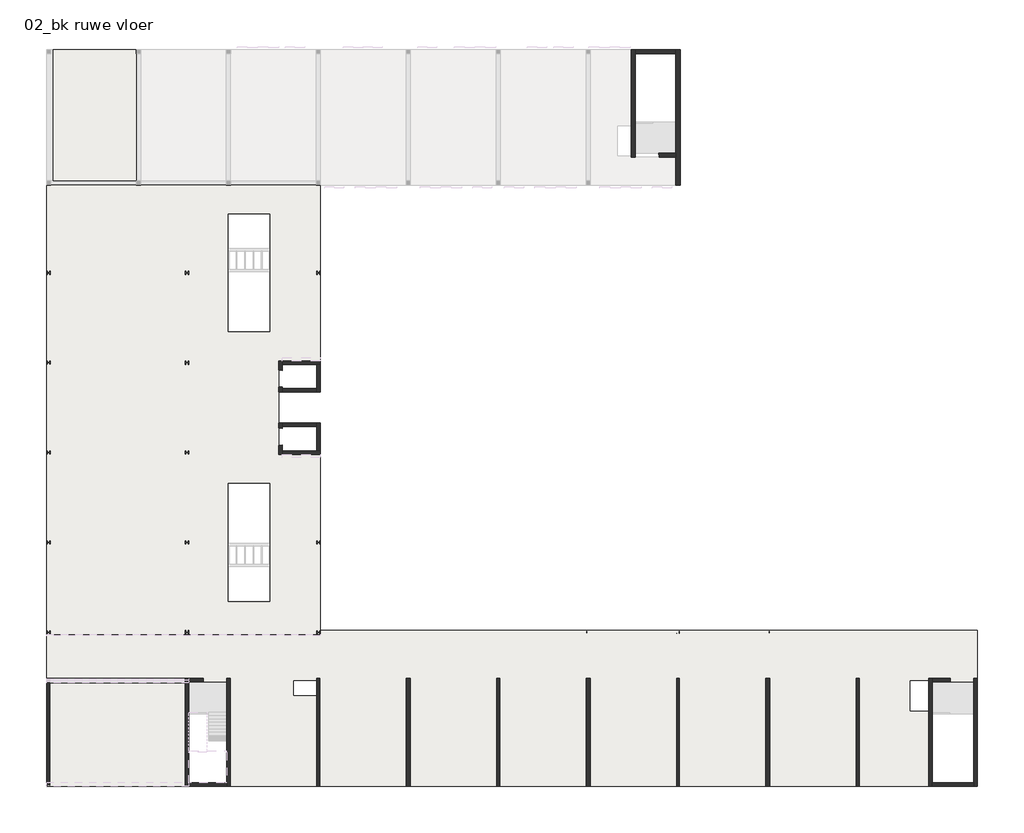
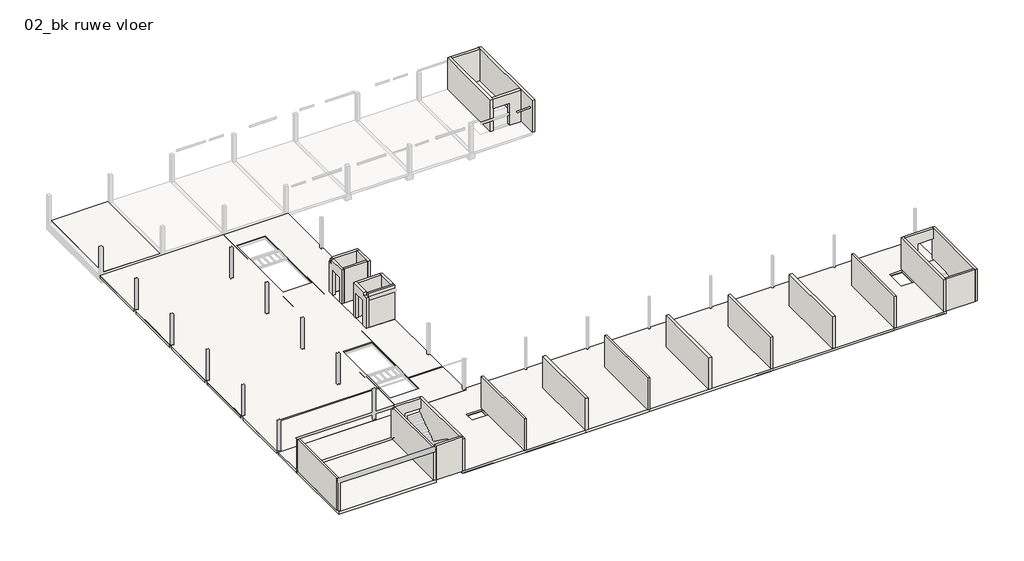
# One storey, part 1 of 3: 28 walls, 20 slabs.
"""IFC4 building model written with IfcOpenShell, lengths in millimetres."""

import ifcopenshell
import ifcopenshell.guid

model = None  # the IFC model being written
_history = None  # IfcOwnerHistory: only IFC2X3 demands one
_inside = {}  # id of a spatial element -> (the spatial element, [elements in it])
_under = {}  # id of a project, library or spatial element -> (it, [spatial elements below it])
_declared = {}  # id of a project -> (the project, [libraries it declares])
_typed = {}  # id of a type object -> (the type object, [elements of that type])
_made_of = {}  # id of a material, layer set ... -> (it, [elements and type objects made of it])


def new_model(schema):
    """Start an empty IFC model of exactly this schema.

    Asked for "IFC4X3", IfcOpenShell would pick the latest addendum, in which some entities
    have other attributes; the version numbers below select the first issue.
    IFC2X3 requires an IfcOwnerHistory on every rooted entity: one is made here for all.
    """
    global model, _history
    if schema == "IFC4X3":
        model = ifcopenshell.file(schema_version=(4, 3, 0, 0))
    else:
        model = ifcopenshell.file(schema=schema)
    _inside.clear()
    _under.clear()
    _declared.clear()
    _typed.clear()
    _made_of.clear()
    _history = None
    if model.schema == "IFC2X3":
        org = make("IfcOrganization", Name="unknown")
        user = make(
            "IfcPersonAndOrganization",
            ThePerson=make("IfcPerson", FamilyName="unknown"),
            TheOrganization=org,
        )
        app = make(
            "IfcApplication",
            ApplicationDeveloper=org,
            Version="unknown",
            ApplicationFullName="unknown",
            ApplicationIdentifier="unknown",
        )
        _history = make(
            "IfcOwnerHistory",
            OwningUser=user,
            OwningApplication=app,
            ChangeAction="ADDED",
            CreationDate=0,
        )
    return model


def make(cls, **values):
    """One entity of the class cls with the attributes given. An attribute that is None is left unset."""
    return model.create_entity(
        cls, **{name: value for name, value in values.items() if value is not None}
    )


def rooted(cls, **values):
    """An entity with a GlobalId (a new one), such as an element, a storey or a relation."""
    return make(cls, GlobalId=ifcopenshell.guid.new(), OwnerHistory=_history, **values)


def si_unit(unit_type, name, prefix=None):
    """IfcSIUnit, for example si_unit("LENGTHUNIT", "METRE", prefix="MILLI")."""
    return make("IfcSIUnit", UnitType=unit_type, Prefix=prefix, Name=name)


def assignment(units):
    """IfcUnitAssignment: the units of a project."""
    return None if units is None else make("IfcUnitAssignment", Units=units)


def point(xyz):
    """IfcCartesianPoint."""
    return None if xyz is None else make("IfcCartesianPoint", Coordinates=xyz)


def direction(xyz):
    """IfcDirection."""
    return None if xyz is None else make("IfcDirection", DirectionRatios=xyz)


def frame(location, z_axis=None, x_axis=None):
    """IfcAxis2Placement3D, a coordinate frame: its origin and axes. An axis left out is left unset."""
    return make(
        "IfcAxis2Placement3D",
        Location=point(location),
        Axis=direction(z_axis),
        RefDirection=direction(x_axis),
    )


def origin():
    """The frame at (0, 0, 0) with its axes left unset."""
    return frame((0.0, 0.0, 0.0))


def place(relative_to, where):
    """IfcLocalPlacement: puts the frame where relative to a parent placement (None: the world)."""
    return make(
        "IfcLocalPlacement", PlacementRelTo=relative_to, RelativePlacement=where
    )


def context(
    kind, dimensions, precision=None, world=None, true_north=None, identifier=None
):
    """IfcGeometricRepresentationContext, for example the 3D "Model" context."""
    return make(
        "IfcGeometricRepresentationContext",
        ContextIdentifier=identifier,
        ContextType=kind,
        CoordinateSpaceDimension=dimensions,
        Precision=precision,
        WorldCoordinateSystem=world,
        TrueNorth=true_north,
    )


def project(units=None, contexts=None):
    """IfcProject with its units and contexts."""
    return rooted(
        "IfcProject",
        Name="project",
        RepresentationContexts=contexts,
        UnitsInContext=assignment(units),
    )


def spatial(cls, under=None, at=None, **own):
    """A site, building, storey or space (cls), placed at a placement, below another one or the project."""
    s = rooted(cls, ObjectPlacement=at, **own)
    if under is not None:
        _under.setdefault(under.id(), (under, []))[1].append(s)
    return s


def polyline(points):
    """IfcPolyline through the points."""
    return make("IfcPolyline", Points=[point(p) for p in points])


def outline(outer, holes=None, kind="AREA"):
    """IfcArbitraryClosedProfileDef: a profile drawn as a closed curve; with holes, ...WithVoids."""
    if holes is None:
        return make("IfcArbitraryClosedProfileDef", ProfileType=kind, OuterCurve=outer)
    return make(
        "IfcArbitraryProfileDefWithVoids",
        ProfileType=kind,
        OuterCurve=outer,
        InnerCurves=holes,
    )


def extrude(swept, where, along, depth):
    """IfcExtrudedAreaSolid: the profile swept, set in the frame where, extruded along a direction by depth."""
    return make(
        "IfcExtrudedAreaSolid",
        SweptArea=swept,
        Position=where,
        ExtrudedDirection=direction(along),
        Depth=depth,
    )


def faces_of(points, faces, orient=None, outer=None):
    """IfcFace entities. A face is a list of loops; a loop is a list of indices into points, from 0.

    orient and outer hold one flag for each loop. By default every Orientation is true, the
    first loop of a face is its IfcFaceOuterBound and the others are IfcFaceBound.
    """
    made = []
    for i, loops in enumerate(faces):
        bounds = []
        for j, loop in enumerate(loops):
            is_outer = j == 0 if outer is None else outer[i][j]
            bounds.append(
                make(
                    "IfcFaceOuterBound" if is_outer else "IfcFaceBound",
                    Bound=make("IfcPolyLoop", Polygon=[points[k] for k in loop]),
                    Orientation=True if orient is None else orient[i][j],
                )
            )
        made.append(make("IfcFace", Bounds=bounds))
    return made


def faceted_brep(points, faces, orient=None, outer=None, voids=None):
    """IfcFacetedBrep: a solid bounded by flat faces; with voids (closed shells), ...WithVoids."""
    shared = [point(p) for p in points]
    hull = make("IfcClosedShell", CfsFaces=faces_of(shared, faces, orient, outer))
    if voids is None:
        return make("IfcFacetedBrep", Outer=hull)
    return make(
        "IfcFacetedBrepWithVoids",
        Outer=hull,
        Voids=[
            make(cls, CfsFaces=faces_of(shared, fs, o, b)) for cls, fs, o, b in voids
        ],
    )


def shape(context_of_items, identifier, shape_type, items):
    """IfcShapeRepresentation: the items that make up one representation, for example the "Body"."""
    return make(
        "IfcShapeRepresentation",
        ContextOfItems=context_of_items,
        RepresentationIdentifier=identifier,
        RepresentationType=shape_type,
        Items=items,
    )


def made_of(thing, what):
    """Note that an element or type object is made of a material, layer set ...; save() writes the relation."""
    if what is not None:
        _made_of.setdefault(what.id(), (what, []))[1].append(thing)
    return thing


def element(
    cls,
    number,
    at=None,
    inside=None,
    cuts=None,
    type_object=None,
    material=None,
    context=None,
    identifier="Body",
    shape_type=None,
    held_by="IfcProductDefinitionShape",
    body=None,
    shapes=None,
    **own,
):
    """One element of the class cls, such as IfcWall. Its Tag is "e" and its number.

    at: its placement. inside: the storey or other place that contains it. cuts: it is an
    opening in that element (IfcRelVoidsElement). A single representation is given by context,
    identifier, shape_type and body (its items); several are given by shapes. held_by: the class
    of the entity that holds the representations. save() writes the other relations.
    """
    e = rooted(cls, Tag="e%d" % number, ObjectPlacement=at, **own)
    if body is not None:
        shapes = [shape(context, identifier, shape_type, body)]
    if shapes is not None:
        e.Representation = make(held_by, Representations=shapes)
    if inside is not None:
        _inside.setdefault(inside.id(), (inside, []))[1].append(e)
    if cuts is not None:
        rooted(
            "IfcRelVoidsElement", RelatingBuildingElement=cuts, RelatedOpeningElement=e
        )
    if type_object is not None:
        _typed.setdefault(type_object.id(), (type_object, []))[1].append(e)
    return made_of(e, material)


def aggregate(whole, parts):
    """IfcRelAggregates: a whole, such as a stair, and the parts it consists of."""
    return rooted("IfcRelAggregates", RelatingObject=whole, RelatedObjects=parts)


def save(model, path):
    """Write the relations noted so far, then the file.

    IfcRelAggregates (storeys below a building ...), IfcRelContainedInSpatialStructure (elements
    in a storey), IfcRelDefinesByType, IfcRelAssociatesMaterial and IfcRelDeclares: one each for
    every whole, place, type object, material and project.
    """
    for whole, parts in _under.values():
        aggregate(whole, parts)
    for where, things in _inside.values():
        rooted(
            "IfcRelContainedInSpatialStructure",
            RelatedElements=things,
            RelatingStructure=where,
        )
    for kind, things in _typed.values():
        rooted("IfcRelDefinesByType", RelatedObjects=things, RelatingType=kind)
    for what, things in _made_of.values():
        rooted("IfcRelAssociatesMaterial", RelatedObjects=things, RelatingMaterial=what)
    for by, libraries in _declared.values():
        rooted("IfcRelDeclares", RelatingContext=by, RelatedDefinitions=libraries)
    model.write(path)


model = new_model("IFC4")

# Units and contexts
model_context = context("Model", 3, world=origin())
ifc_project = project(units=[si_unit("LENGTHUNIT", "METRE", prefix="MILLI")], contexts=[model_context])

# Site, building, storey
site = spatial("IfcSite", under=ifc_project)
building = spatial("IfcBuilding", under=site)
storey = spatial("IfcBuildingStorey", under=building, Name="02_bk ruwe vloer", Elevation=7530.0)

# Slabs
placement = place(None, origin())
element("IfcSlab", 1, ObjectType="NLRS_23_FL_breedplaat 260_gen_rsf", at=placement, inside=storey, context=model_context, shape_type="Brep", body=[
    faceted_brep([(70375.0, -150.0, 7270.0), (70125.0, -150.0, 7270.0), (65150.0, -150.0, 7270.0), (64850.0, -150.0, 7270.0), (58650.0, -150.0, 7270.0), (58350.0, -150.0, 7270.0), (52150.0, -150.0, 7270.0), (51850.0, -150.0, 7270.0), (45650.0, -150.0, 7270.0), (45350.0, -150.0, 7270.0), (39150.0, -150.0, 7270.0), (38850.0, -150.0, 7270.0), (32650.0, -150.0, 7270.0), (32350.0, -150.0, 7270.0), (19625.0, -150.0, 7270.0), (19375.0, -150.0, 7270.0), (19375.0, 7400.0, 7270.0), (16625.0, 7400.0, 7270.0), (16625.0, 7493.0, 7270.0), (16625.0, 7507.0, 7270.0), (6350.0, 7507.0, 7270.0), (6350.0, 10845.0, 7270.0), (26125.0, 10845.0, 7270.0), (26125.0, 11125.0, 7270.0), (73650.0, 11125.0, 7270.0), (73650.0, 7400.0, 7270.0), (73400.0, 7400.0, 7270.0), (70375.0, 7400.0, 7270.0), (6370.0, 7622.0, 7270.0), (19600.0, 7622.0, 7270.0), (19600.0, -130.0, 7270.0), (25875.0, -130.0, 7270.0), (25875.0, 7625.0, 7270.0), (26125.0, 7625.0, 7270.0), (26125.0, -130.0, 7270.0), (32375.0, -130.0, 7270.0), (32375.0, 125.0, 7270.0), (32625.0, 125.0, 7270.0), (32625.0, -130.0, 7270.0), (38875.0, -130.0, 7270.0), (38875.0, 7625.0, 7270.0), (39125.0, 7625.0, 7270.0), (39125.0, -130.0, 7270.0), (45375.0, -130.0, 7270.0), (45375.0, 125.0, 7270.0), (45625.0, 125.0, 7270.0), (45625.0, -130.0, 7270.0), (51875.0, -130.0, 7270.0), (51875.0, 7625.0, 7270.0), (52125.0, 7625.0, 7270.0), (52125.0, -130.0, 7270.0), (58375.0, -130.0, 7270.0), (58375.0, 125.0, 7270.0), (58625.0, 125.0, 7270.0), (58625.0, -130.0, 7270.0), (64875.0, -130.0, 7270.0), (64875.0, 7625.0, 7270.0), (65125.0, 7625.0, 7270.0), (65125.0, -130.0, 7270.0), (70150.0, -130.0, 7270.0), (70150.0, 7625.0, 7270.0), (73630.0, 7625.0, 7270.0), (73630.0, 11105.0, 7270.0), (26145.0, 11105.0, 7270.0), (26145.0, 10761.5, 7270.0), (6370.0, 10761.5, 7270.0), (32375.0, 7625.0, 7270.0), (32625.0, 7625.0, 7270.0), (32625.0, 7375.0, 7270.0), (32375.0, 7375.0, 7270.0), (45375.0, 7625.0, 7270.0), (45625.0, 7625.0, 7270.0), (45625.0, 7375.0, 7270.0), (45375.0, 7375.0, 7270.0), (58375.0, 7625.0, 7270.0), (58625.0, 7625.0, 7270.0), (58625.0, 7375.0, 7270.0), (58375.0, 7375.0, 7270.0), (19375.0, -150.0, 7530.0), (19625.0, -150.0, 7530.0), (32350.0, -150.0, 7530.0), (32650.0, -150.0, 7530.0), (45350.0, -150.0, 7530.0), (45650.0, -150.0, 7530.0), (58350.0, -150.0, 7530.0), (58650.0, -150.0, 7530.0), (70125.0, -150.0, 7530.0), (70375.0, -150.0, 7530.0), (70375.0, 7400.0, 7530.0), (71700.0, 7400.0, 7530.0), (73650.0, 7400.0, 7530.0), (73650.0, 11125.0, 7530.0), (26125.0, 11125.0, 7530.0), (26125.0, 10845.0, 7530.0), (6350.0, 10845.0, 7530.0), (6350.0, 7507.0, 7530.0), (16625.0, 7507.0, 7530.0), (16625.0, 7493.0, 7530.0), (16625.0, 7400.0, 7530.0), (19375.0, 7400.0, 7530.0), (19375.0, 100.0, 7530.0), (24227.5, 6452.0, 7530.0), (24227.5, 7500.0, 7530.0), (25850.0, 7500.0, 7530.0), (25850.0, 6452.0, 7530.0), (68805.0, 5320.0, 7530.0), (68805.0, 7500.0, 7530.0), (70125.0, 7500.0, 7530.0), (70125.0, 5320.0, 7530.0), (6350.0, 10845.0, 7480.0), (26125.0, 10845.0, 7480.0), (19600.0, 7622.0, 7330.0), (6370.0, 7622.0, 7330.0), (6370.0, 10761.5, 7330.0), (26145.0, 10761.5, 7330.0), (26145.0, 11105.0, 7330.0), (73630.0, 11105.0, 7330.0), (73630.0, 7625.0, 7330.0), (70150.0, 7625.0, 7330.0), (70150.0, -130.0, 7330.0), (65125.0, -130.0, 7330.0), (65125.0, 7625.0, 7330.0), (64875.0, 7625.0, 7330.0), (64875.0, -130.0, 7330.0), (58625.0, -130.0, 7330.0), (58625.0, 125.0, 7330.0), (58375.0, 125.0, 7330.0), (58375.0, -130.0, 7330.0), (52125.0, -130.0, 7330.0), (52125.0, 7625.0, 7330.0), (51875.0, 7625.0, 7330.0), (51875.0, -130.0, 7330.0), (45625.0, -130.0, 7330.0), (45625.0, 125.0, 7330.0), (45375.0, 125.0, 7330.0), (45375.0, -130.0, 7330.0), (39125.0, -130.0, 7330.0), (39125.0, 7625.0, 7330.0), (38875.0, 7625.0, 7330.0), (38875.0, -130.0, 7330.0), (32625.0, -130.0, 7330.0), (32625.0, 125.0, 7330.0), (32375.0, 125.0, 7330.0), (32375.0, -130.0, 7330.0), (26125.0, -130.0, 7330.0), (26125.0, 7625.0, 7330.0), (25875.0, 7625.0, 7330.0), (25875.0, -130.0, 7330.0), (19600.0, -130.0, 7330.0), (32625.0, 7625.0, 7330.0), (32375.0, 7625.0, 7330.0), (32375.0, 7375.0, 7330.0), (32625.0, 7375.0, 7330.0), (45625.0, 7625.0, 7330.0), (45375.0, 7625.0, 7330.0), (45375.0, 7375.0, 7330.0), (45625.0, 7375.0, 7330.0), (58625.0, 7625.0, 7330.0), (58375.0, 7625.0, 7330.0), (58375.0, 7375.0, 7330.0), (58625.0, 7375.0, 7330.0), (24227.5, 7500.0, 7330.0), (24227.5, 6452.0, 7330.0), (25850.0, 6452.0, 7330.0), (25850.0, 7500.0, 7330.0), (68805.0, 7500.0, 7330.0), (68805.0, 5320.0, 7330.0), (70125.0, 5320.0, 7330.0), (70125.0, 7500.0, 7330.0)], [[[0, 1, 2, 3, 4, 5, 6, 7, 8, 9, 10, 11, 12, 13, 14, 15, 16, 17, 18, 19, 20, 21, 22, 23, 24, 25, 26, 27], [28, 29, 30, 31, 32, 33, 34, 35, 36, 37, 38, 39, 40, 41, 42, 43, 44, 45, 46, 47, 48, 49, 50, 51, 52, 53, 54, 55, 56, 57, 58, 59, 60, 61, 62, 63, 64, 65]], [[66, 67, 68, 69]], [[70, 71, 72, 73]], [[74, 75, 76, 77]], [[78, 79, 80, 81, 82, 83, 84, 85, 86, 87, 88, 89, 90, 91, 92, 93, 94, 95, 96, 97, 98, 99, 100], [101, 102, 103, 104], [105, 106, 107, 108]], [[15, 14, 13, 12, 11, 10, 9, 8, 7, 6, 5, 4, 3, 2, 1, 0, 87, 86, 85, 84, 83, 82, 81, 80, 79, 78]], [[16, 15, 78, 100, 99]], [[17, 16, 99, 98]], [[17, 98, 97, 96, 19, 18]], [[21, 20, 95, 94, 109]], [[22, 21, 109, 94, 93, 110]], [[23, 22, 110, 93, 92]], [[24, 23, 92, 91]], [[25, 24, 91, 90]], [[27, 26, 25, 90, 89, 88]], [[0, 27, 88, 87]], [[20, 19, 96, 95]], [[111, 112, 113, 114, 115, 116, 117, 118, 119, 120, 121, 122, 123, 124, 125, 126, 127, 128, 129, 130, 131, 132, 133, 134, 135, 136, 137, 138, 139, 140, 141, 142, 143, 144, 145, 146, 147, 148], [149, 150, 151, 152], [153, 154, 155, 156], [157, 158, 159, 160], [161, 162, 163, 164], [165, 166, 167, 168]], [[112, 111, 29, 28]], [[113, 112, 28, 65]], [[114, 113, 65, 64]], [[115, 114, 64, 63]], [[116, 115, 63, 62]], [[117, 116, 62, 61]], [[118, 117, 61, 60]], [[119, 118, 60, 59]], [[120, 119, 59, 58]], [[121, 120, 58, 57]], [[122, 121, 57, 56]], [[123, 122, 56, 55]], [[124, 123, 55, 54]], [[125, 124, 54, 53]], [[126, 125, 53, 52]], [[127, 126, 52, 51]], [[128, 127, 51, 50]], [[129, 128, 50, 49]], [[130, 129, 49, 48]], [[131, 130, 48, 47]], [[132, 131, 47, 46]], [[133, 132, 46, 45]], [[134, 133, 45, 44]], [[135, 134, 44, 43]], [[136, 135, 43, 42]], [[137, 136, 42, 41]], [[138, 137, 41, 40]], [[139, 138, 40, 39]], [[140, 139, 39, 38]], [[141, 140, 38, 37]], [[142, 141, 37, 36]], [[143, 142, 36, 35]], [[144, 143, 35, 34]], [[145, 144, 34, 33]], [[146, 145, 33, 32]], [[147, 146, 32, 31]], [[148, 147, 31, 30]], [[111, 148, 30, 29]], [[150, 149, 67, 66]], [[151, 150, 66, 69]], [[152, 151, 69, 68]], [[149, 152, 68, 67]], [[154, 153, 71, 70]], [[155, 154, 70, 73]], [[156, 155, 73, 72]], [[153, 156, 72, 71]], [[158, 157, 75, 74]], [[159, 158, 74, 77]], [[160, 159, 77, 76]], [[157, 160, 76, 75]], [[102, 101, 162, 161]], [[101, 104, 163, 162]], [[104, 103, 164, 163]], [[103, 102, 161, 164]], [[106, 105, 166, 165]], [[105, 108, 167, 166]], [[108, 107, 168, 167]], [[107, 106, 165, 168]]]),
])
element("IfcSlab", 2, ObjectType="NLRS_23_FL_breedplaat 260_gen_rsf", at=placement, inside=storey, context=model_context, shape_type="Brep", body=[
    faceted_brep([(6830.0, 43680.0, 7270.0), (6830.0, 43800.0, 7270.0), (6830.0, 53150.0, 7270.0), (6950.0, 53150.0, 7270.0), (12700.0, 53150.0, 7270.0), (12820.0, 53150.0, 7270.0), (12820.0, 43800.0, 7270.0), (12820.0, 43680.0, 7270.0), (12725.0, 43775.0, 7270.0), (12725.0, 53140.0, 7270.0), (6925.0, 53140.0, 7270.0), (6925.0, 43775.0, 7270.0), (6830.0, 53150.0, 7530.0), (6830.0, 43680.0, 7530.0), (12820.0, 43680.0, 7530.0), (12820.0, 53150.0, 7530.0), (6925.0, 53140.0, 7330.0), (12725.0, 53140.0, 7330.0), (12725.0, 43775.0, 7330.0), (6925.0, 43775.0, 7330.0)], [[[0, 1, 2, 3, 4, 5, 6, 7], [8, 9, 10, 11]], [[12, 13, 14, 15]], [[2, 1, 0, 13, 12]], [[5, 4, 3, 2, 12, 15]], [[7, 6, 5, 15, 14]], [[0, 7, 14, 13]], [[16, 17, 18, 19]], [[18, 17, 9, 8]], [[19, 18, 8, 11]], [[16, 19, 11, 10]], [[17, 16, 10, 9]]]),
])
element("IfcSlab", 3, ObjectType="NLRS_23_FL_druklaag 70_gen_rsf", at=placement, inside=storey, context=model_context, shape_type="Brep", body=[
    faceted_brep([(6350.0, 43350.0, 7460.0), (26125.0, 43350.0, 7460.0), (26125.0, 43330.0, 7460.0), (26125.0, 37175.0, 7460.0), (26125.0, 37155.0, 7460.0), (22760.0, 37155.0, 7460.0), (22760.0, 36845.0, 7460.0), (26125.0, 36845.0, 7460.0), (26125.0, 36825.0, 7460.0), (26125.0, 30705.0, 7460.0), (26125.0, 30625.0, 7460.0), (23362.3, 30625.0, 7460.0), (23362.3, 30632.0, 7460.0), (6350.0, 30632.0, 7460.0), (6350.0, 30652.0, 7460.0), (6350.0, 36825.0, 7460.0), (6350.0, 36845.0, 7460.0), (19240.0, 36845.0, 7460.0), (19240.0, 37155.0, 7460.0), (6350.0, 37155.0, 7460.0), (6350.0, 37175.0, 7460.0), (6350.0, 43330.0, 7460.0), (22500.0, 32750.0, 7460.0), (22500.0, 41250.0, 7460.0), (19500.0, 41250.0, 7460.0), (19500.0, 32750.0, 7460.0), (23362.3, 23875.0, 7460.0), (26125.0, 23875.0, 7460.0), (26125.0, 23795.0, 7460.0), (26125.0, 17675.0, 7460.0), (26125.0, 17655.0, 7460.0), (26125.0, 17345.0, 7460.0), (26125.0, 17325.0, 7460.0), (26125.0, 11175.0, 7460.0), (26125.0, 11155.0, 7460.0), (6350.0, 11155.0, 7460.0), (6350.0, 11175.0, 7460.0), (6350.0, 17325.0, 7460.0), (6350.0, 17345.0, 7460.0), (19240.0, 17345.0, 7460.0), (19240.0, 17655.0, 7460.0), (6350.0, 17655.0, 7460.0), (6350.0, 17675.0, 7460.0), (6350.0, 23825.0, 7460.0), (6350.0, 23845.0, 7460.0), (19240.0, 23845.0, 7460.0), (19500.0, 23845.0, 7460.0), (22500.0, 23845.0, 7460.0), (22760.0, 23845.0, 7460.0), (23362.3, 23845.0, 7460.0), (22500.0, 21750.0, 7460.0), (19500.0, 21750.0, 7460.0), (19500.0, 13250.0, 7460.0), (22500.0, 13250.0, 7460.0), (19500.0000006, 13240.0, 7460.0), (19500.0000006, 12938.0, 7460.0), (22499.9999994, 12938.0, 7460.0), (22499.9999994, 13240.0, 7460.0), (19500.0000006, 22062.0, 7460.0), (19500.0000006, 21760.0, 7460.0), (22499.9999994, 21760.0, 7460.0), (22499.9999994, 22062.0, 7460.0), (6350.0, 30322.0, 7460.0), (23125.0, 30322.0, 7460.0), (23125.0, 30302.0, 7460.0), (23125.0, 24175.0, 7460.0), (23125.0, 24155.0, 7460.0), (6350.0, 24155.0, 7460.0), (6350.0, 24175.0, 7460.0), (6350.0, 30302.0, 7460.0), (26125.0, 30625.0, 7530.0), (26125.0, 43350.0, 7530.0), (6350.0, 43350.0, 7530.0), (6350.0, 10845.0, 7530.0), (26125.0, 10845.0, 7530.0), (26125.0, 11125.0, 7530.0), (26125.0, 23875.0, 7530.0), (23125.0, 23875.0, 7530.0), (23125.0, 30625.0, 7530.0), (22500.0, 41250.0, 7530.0), (22500.0, 32750.0, 7530.0), (19500.0, 32750.0, 7530.0), (19500.0, 41250.0, 7530.0), (19500.0, 21750.0, 7530.0), (22500.0, 21750.0, 7530.0), (22500.0, 13250.0, 7530.0), (19500.0, 13250.0, 7530.0), (26125.0, 36845.0, 7480.0), (26125.0, 37155.0, 7480.0), (6350.0, 10845.0, 7480.0), (26125.0, 10845.0, 7480.0), (6350.0, 37155.0, 7480.0), (6350.0, 36845.0, 7480.0), (6350.0, 30632.0, 7480.0), (6350.0, 30322.0, 7480.0), (6350.0, 24155.0, 7480.0), (6350.0, 23845.0, 7480.0), (6350.0, 17655.0, 7480.0), (6350.0, 17345.0, 7480.0), (6350.0, 11155.0, 7480.0), (23125.0, 30625.0, 7480.0), (23362.3, 30625.0, 7480.0), (23125.0, 23875.0, 7480.0), (23125.0, 24155.0, 7480.0), (23125.0, 30322.0, 7480.0), (23362.3, 23875.0, 7480.0), (26125.0, 11125.0, 7480.0), (26125.0, 11155.0, 7480.0), (19240.0, 36845.0, 7480.0), (19240.0, 37155.0, 7480.0), (23362.3, 30632.0, 7480.0), (23362.3, 23845.0, 7480.0), (19240.0, 17345.0, 7480.0), (19240.0, 17655.0, 7480.0), (22760.0, 37155.0, 7480.0), (22760.0, 36845.0, 7480.0), (19500.0000006, 13240.0, 7480.0), (19500.0000006, 12938.0, 7480.0), (22499.9999994, 12938.0, 7480.0), (22499.9999994, 13240.0, 7480.0), (19500.0000006, 22062.0, 7480.0), (19500.0000006, 21760.0, 7480.0), (22499.9999994, 21760.0, 7480.0), (22499.9999994, 22062.0, 7480.0)], [[[0, 1, 2, 3, 4, 5, 6, 7, 8, 9, 10, 11, 12, 13, 14, 15, 16, 17, 18, 19, 20, 21], [22, 23, 24, 25]], [[26, 27, 28, 29, 30, 31, 32, 33, 34, 35, 36, 37, 38, 39, 40, 41, 42, 43, 44, 45, 46, 47, 48, 49], [50, 51, 52, 53], [54, 55, 56, 57], [58, 59, 60, 61]], [[62, 63, 64, 65, 66, 67, 68, 69]], [[70, 71, 72, 73, 74, 75, 76, 77, 78], [79, 80, 81, 82], [83, 84, 85, 86]], [[71, 70, 10, 9, 8, 7, 87, 88, 4, 3, 2, 1]], [[74, 73, 89, 90]], [[73, 72, 0, 21, 20, 19, 91, 92, 16, 15, 14, 13, 93, 94, 62, 69, 68, 67, 95, 96, 44, 43, 42, 41, 97, 98, 38, 37, 36, 35, 99, 89]], [[1, 0, 72, 71]], [[70, 78, 100, 101, 11, 10]], [[78, 77, 102, 103, 66, 65, 64, 63, 104, 100]], [[77, 76, 27, 26, 105, 102]], [[27, 76, 75, 74, 90, 106, 107, 34, 33, 32, 31, 30, 29, 28]], [[23, 22, 80, 79]], [[24, 23, 79, 82]], [[25, 24, 82, 81]], [[22, 25, 81, 80]], [[51, 50, 84, 83]], [[52, 51, 83, 86]], [[53, 52, 86, 85]], [[50, 53, 85, 84]], [[108, 109, 18, 17]], [[109, 108, 92, 91]], [[109, 91, 19, 18]], [[92, 108, 17, 16]], [[101, 110, 12, 11]], [[93, 110, 101, 100, 104, 94]], [[110, 93, 13, 12]], [[94, 104, 63, 62]], [[111, 105, 26, 49]], [[111, 96, 95, 103, 102, 105]], [[103, 95, 67, 66]], [[96, 111, 49, 48, 47, 46, 45, 44]], [[112, 113, 40, 39]], [[113, 112, 98, 97]], [[113, 97, 41, 40]], [[98, 112, 39, 38]], [[99, 107, 106, 90, 89]], [[107, 99, 35, 34]], [[114, 115, 6, 5]], [[115, 114, 88, 87]], [[88, 114, 5, 4]], [[115, 87, 7, 6]], [[116, 117, 55, 54]], [[118, 119, 57, 56]], [[117, 116, 119, 118]], [[119, 116, 54, 57]], [[117, 118, 56, 55]], [[120, 121, 59, 58]], [[122, 123, 61, 60]], [[121, 120, 123, 122]], [[121, 122, 60, 59]], [[123, 120, 58, 61]]]),
])
element("IfcSlab", 4, ObjectType="NLRS_23_FL_kanaalplaat 260_gen_rsf", at=placement, inside=storey, context=model_context, shape_type="SweptSolid", body=[
    extrude(outline(polyline([(19240.0, 11175.0), (6350.0, 11175.0), (6350.0, 17325.0), (19240.0, 17325.0), (19240.0, 11175.0)])), frame((0.0, 0.0, 7200.0), z_axis=(0.0, 0.0, 1.0), x_axis=(1.0, 0.0, 0.0)), (0.0, 0.0, 1.0), 260.0),
])
element("IfcSlab", 5, ObjectType="NLRS_23_FL_kanaalplaat 260_gen_rsf", at=placement, inside=storey, context=model_context, shape_type="SweptSolid", body=[
    extrude(outline(polyline([(6350.0, 17675.0), (6350.0, 23825.0), (19240.0, 23825.0), (19240.0, 17675.0), (6350.0, 17675.0)])), frame((0.0, 0.0, 7200.0), z_axis=(0.0, 0.0, 1.0), x_axis=(1.0, 0.0, 0.0)), (0.0, 0.0, 1.0), 260.0),
])
element("IfcSlab", 6, ObjectType="NLRS_23_FL_kanaalplaat 260_gen_rsf", at=placement, inside=storey, context=model_context, shape_type="SweptSolid", body=[
    extrude(outline(polyline([(23125.0, 30302.0), (23125.0, 24175.0), (6350.0, 24175.0), (6350.0, 30302.0), (23125.0, 30302.0)])), frame((0.0, 0.0, 7200.0), z_axis=(0.0, 0.0, 1.0), x_axis=(1.0, 0.0, 0.0)), (0.0, 0.0, 1.0), 260.0),
])
element("IfcSlab", 7, ObjectType="NLRS_23_FL_kanaalplaat 260_gen_rsf", at=placement, inside=storey, context=model_context, shape_type="SweptSolid", body=[
    extrude(outline(polyline([(22500.0, 23825.0), (22500.0, 22082.0), (19500.0, 22082.0), (19500.0, 23825.0), (22500.0, 23825.0)])), frame((0.0, 0.0, 7200.0), z_axis=(0.0, 0.0, 1.0), x_axis=(1.0, 0.0, 0.0)), (0.0, 0.0, 1.0), 260.0),
])
element("IfcSlab", 8, ObjectType="NLRS_23_FL_kanaalplaat 260_gen_rsf", at=placement, inside=storey, context=model_context, shape_type="SweptSolid", body=[
    extrude(outline(polyline([(22500.0, 11182.5), (19500.0, 11182.5), (19500.0, 12918.0), (22500.0, 12918.0), (22500.0, 11182.5)])), frame((0.0, 0.0, 7200.0), z_axis=(0.0, 0.0, 1.0), x_axis=(1.0, 0.0, 0.0)), (0.0, 0.0, 1.0), 260.0),
])
element("IfcSlab", 9, ObjectType="NLRS_23_FL_kanaalplaat 260_gen_rsf", at=placement, inside=storey, context=model_context, shape_type="Brep", body=[
    faceted_brep([(26125.0, 23795.0, 7200.0), (26125.0, 23625.0, 7200.0), (26125.0, 17675.0, 7200.0), (22760.0, 17675.0, 7200.0), (22760.0, 23825.0, 7200.0), (23395.0, 23825.0, 7200.0), (23395.0, 23795.0, 7200.0), (26125.0, 23795.0, 7460.0), (23395.0, 23795.0, 7460.0), (23395.0, 23825.0, 7460.0), (22760.0, 23825.0, 7460.0), (22760.0, 17675.0, 7460.0), (26125.0, 17675.0, 7460.0)], [[[0, 1, 2, 3, 4, 5, 6]], [[7, 8, 9, 10, 11, 12]], [[2, 1, 0, 7, 12]], [[3, 2, 12, 11]], [[4, 3, 11, 10]], [[5, 4, 10, 9]], [[6, 5, 9, 8]], [[0, 6, 8, 7]]]),
])
element("IfcSlab", 10, ObjectType="NLRS_23_FL_kanaalplaat 260_gen_rsf", at=placement, inside=storey, context=model_context, shape_type="SweptSolid", body=[
    extrude(outline(polyline([(22760.0, 11175.0), (22760.0, 17325.0), (26125.0, 17325.0), (26125.0, 11175.0), (22760.0, 11175.0)])), frame((0.0, 0.0, 7200.0), z_axis=(0.0, 0.0, 1.0), x_axis=(1.0, 0.0, 0.0)), (0.0, 0.0, 1.0), 260.0),
])
element("IfcSlab", 11, ObjectType="NLRS_23_FL_kanaalplaat 260_gen_rsf", at=placement, inside=storey, context=model_context, shape_type="Brep", body=[
    faceted_brep([(19240.0, 43330.0, 7200.0), (19240.0, 37175.0, 7200.0), (6350.0, 37175.0, 7200.0), (6350.0, 43200.0, 7200.0), (6350.0, 43330.0, 7200.0), (19240.0, 43330.0, 7460.0), (6350.0, 43330.0, 7460.0), (6350.0, 37175.0, 7460.0), (19240.0, 37175.0, 7460.0)], [[[0, 1, 2, 3, 4]], [[5, 6, 7, 8]], [[0, 4, 6, 5]], [[4, 3, 2, 7, 6]], [[2, 1, 8, 7]], [[1, 0, 5, 8]]]),
])
element("IfcSlab", 12, ObjectType="NLRS_23_FL_kanaalplaat 260_gen_rsf", at=placement, inside=storey, context=model_context, shape_type="SweptSolid", body=[
    extrude(outline(polyline([(6350.0, 36825.0), (19240.0, 36825.0), (19240.0, 30652.0), (6350.0, 30652.0), (6350.0, 36825.0)])), frame((0.0, 0.0, 7200.0), z_axis=(0.0, 0.0, 1.0), x_axis=(1.0, 0.0, 0.0)), (0.0, 0.0, 1.0), 260.0),
])
element("IfcSlab", 13, ObjectType="NLRS_23_FL_kanaalplaat 260_gen_rsf", at=placement, inside=storey, context=model_context, shape_type="SweptSolid", body=[
    extrude(outline(polyline([(22500.0, 30652.0), (19500.0, 30652.0), (19500.0, 32418.0), (22500.0, 32418.0), (22500.0, 30652.0)])), frame((0.0, 0.0, 7200.0), z_axis=(0.0, 0.0, 1.0), x_axis=(1.0, 0.0, 0.0)), (0.0, 0.0, 1.0), 260.0),
])
element("IfcSlab", 14, ObjectType="NLRS_23_FL_kanaalplaat 260_gen_rsf", at=placement, inside=storey, context=model_context, shape_type="SweptSolid", body=[
    extrude(outline(polyline([(22500.0, 43330.0), (22500.0, 41605.0), (19500.0, 41605.0), (19500.0, 43330.0), (22500.0, 43330.0)])), frame((0.0, 0.0, 7200.0), z_axis=(0.0, 0.0, 1.0), x_axis=(1.0, 0.0, 0.0)), (0.0, 0.0, 1.0), 260.0),
])
element("IfcSlab", 15, ObjectType="NLRS_23_FL_kanaalplaat 260_gen_rsf", at=placement, inside=storey, context=model_context, shape_type="Brep", body=[
    faceted_brep([(26125.0, 30705.0, 7200.0), (23395.0, 30705.0, 7200.0), (23395.0, 30652.0, 7200.0), (22760.0, 30652.0, 7200.0), (22760.0, 36825.0, 7200.0), (26125.0, 36825.0, 7200.0), (26125.0, 30875.0, 7200.0), (26125.0, 30705.0, 7460.0), (26125.0, 36825.0, 7460.0), (22760.0, 36825.0, 7460.0), (22760.0, 30652.0, 7460.0), (23395.0, 30652.0, 7460.0), (23395.0, 30705.0, 7460.0)], [[[0, 1, 2, 3, 4, 5, 6]], [[7, 8, 9, 10, 11, 12]], [[0, 6, 5, 8, 7]], [[5, 4, 9, 8]], [[4, 3, 10, 9]], [[3, 2, 11, 10]], [[2, 1, 12, 11]], [[1, 0, 7, 12]]]),
])
element("IfcSlab", 16, ObjectType="NLRS_23_FL_kanaalplaat 260_gen_rsf", at=placement, inside=storey, context=model_context, shape_type="Brep", body=[
    faceted_brep([(22760.0, 43330.0, 7200.0), (26125.0, 43330.0, 7200.0), (26125.0, 43200.0, 7200.0), (26125.0, 37175.0, 7200.0), (22760.0, 37175.0, 7200.0), (22760.0, 43330.0, 7460.0), (22760.0, 37175.0, 7460.0), (26125.0, 37175.0, 7460.0), (26125.0, 43330.0, 7460.0)], [[[0, 1, 2, 3, 4]], [[5, 6, 7, 8]], [[0, 4, 6, 5]], [[4, 3, 7, 6]], [[3, 2, 1, 8, 7]], [[1, 0, 5, 8]]]),
])
element("IfcSlab", 17, ObjectType="NLRS_23_FL_breedplaat 260_gen_rsf", at=placement, inside=storey, context=model_context, shape_type="Brep", body=[
    faceted_brep([(6350.0, -150.0, 7270.0), (6350.0, 7493.0, 7270.0), (16625.0, 7493.0, 7270.0), (16625.0, 7330.0, 7270.0), (16625.0, 170.0, 7270.0), (16625.0, -150.0, 7270.0), (16400.0, 125.0, 7270.0), (16400.0, 7378.0, 7270.0), (6539.0, 7378.0, 7270.0), (6539.0, 125.0, 7270.0), (6350.0, 7493.0, 7530.0), (6350.0, -150.0, 7530.0), (16375.0, -150.0, 7530.0), (16625.0, -150.0, 7530.0), (16625.0, 100.0, 7530.0), (16625.0, 7493.0, 7530.0), (6539.0, 7378.0, 7330.0), (16400.0, 7378.0, 7330.0), (16400.0, 125.0, 7330.0), (6539.0, 125.0, 7330.0)], [[[0, 1, 2, 3, 4, 5], [6, 7, 8, 9]], [[10, 11, 12, 13, 14, 15]], [[1, 0, 11, 10]], [[2, 1, 10, 15]], [[5, 4, 3, 2, 15, 14, 13]], [[0, 5, 13, 12, 11]], [[16, 17, 18, 19]], [[18, 17, 7, 6]], [[19, 18, 6, 9]], [[16, 19, 9, 8]], [[17, 16, 8, 7]]]),
])
element("IfcSlab", 18, ObjectType="NLRS_23_FL_breedplaat schil 60_gen_rsf", at=placement, inside=storey, context=model_context, shape_type="SweptSolid", body=[
    extrude(outline(polyline([(19600.0, 7622.0), (6370.0, 7622.0), (6370.0, 10761.5), (26145.0, 10761.5), (26145.0, 11105.0), (73630.0, 11105.0), (73630.0, 7625.0), (70150.0, 7625.0), (70150.0, -130.0), (65125.0, -130.0), (65125.0, 7625.0), (64875.0, 7625.0), (64875.0, -130.0), (58625.0, -130.0), (58625.0, 125.0), (58375.0, 125.0), (58375.0, -130.0), (52125.0, -130.0), (52125.0, 7625.0), (51875.0, 7625.0), (51875.0, -130.0), (45625.0, -130.0), (45625.0, 125.0), (45375.0, 125.0), (45375.0, -130.0), (39125.0, -130.0), (39125.0, 7625.0), (38875.0, 7625.0), (38875.0, -130.0), (32625.0, -130.0), (32625.0, 125.0), (32375.0, 125.0), (32375.0, -130.0), (26125.0, -130.0), (26125.0, 7625.0), (25875.0, 7625.0), (25875.0, -130.0), (19600.0, -130.0), (19600.0, 7622.0)]), holes=[polyline([(32625.0, 7625.0), (32375.0, 7625.0), (32375.0, 7375.0), (32625.0, 7375.0), (32625.0, 7625.0)]), polyline([(45625.0, 7625.0), (45375.0, 7625.0), (45375.0, 7375.0), (45625.0, 7375.0), (45625.0, 7625.0)]), polyline([(58625.0, 7625.0), (58375.0, 7625.0), (58375.0, 7375.0), (58625.0, 7375.0), (58625.0, 7625.0)]), polyline([(24227.5, 7500.0), (24227.5, 6452.0), (25850.0, 6452.0), (25850.0, 7500.0), (24227.5, 7500.0)]), polyline([(68805.0, 7500.0), (68805.0, 5320.0), (70125.0, 5320.0), (70125.0, 7500.0), (68805.0, 7500.0)])]), frame((0.0, 0.0, 7270.0), z_axis=(0.0, 0.0, 1.0), x_axis=(1.0, 0.0, 0.0)), (0.0, 0.0, 1.0), 60.0),
])
element("IfcSlab", 19, ObjectType="NLRS_23_FL_breedplaat schil 60_gen_rsf", at=placement, inside=storey, context=model_context, shape_type="SweptSolid", body=[
    extrude(outline(polyline([(16400.0, 7378.0), (16400.0, 125.0), (6539.0, 125.0), (6539.0, 7378.0), (16400.0, 7378.0)])), frame((0.0, 0.0, 7270.0), z_axis=(0.0, 0.0, 1.0), x_axis=(1.0, 0.0, 0.0)), (0.0, 0.0, 1.0), 60.0),
])
element("IfcSlab", 20, ObjectType="NLRS_23_FL_breedplaat schil 60_gen_rsf", at=placement, inside=storey, context=model_context, shape_type="SweptSolid", body=[
    extrude(outline(polyline([(12725.0, 53140.0), (12725.0, 43775.0), (6925.0, 43775.0), (6925.0, 53140.0), (12725.0, 53140.0)])), frame((0.0, 0.0, 7270.0), z_axis=(0.0, 0.0, 1.0), x_axis=(1.0, 0.0, 0.0)), (0.0, 0.0, 1.0), 60.0),
])

# Walls
element("IfcWall", 21, ObjectType="NLRS_22_WA_beton ihw 250_gen_rsf", at=placement, inside=storey, context=model_context, shape_type="Brep", body=[
    faceted_brep([(19625.0, -150.0, 7530.0), (19625.0, 7650.0, 7530.0), (19625.0, 7650.0, 11070.0), (19625.0, -150.0, 11070.0), (19375.0, -150.0, 7530.0), (19375.0, -150.0, 11070.0), (19375.0, 7400.0, 11070.0), (19375.0, 7650.0, 11070.0), (19375.0, 7650.0, 9970.0), (19375.0, 7650.0, 7530.0), (19375.0, 7400.0, 7530.0), (19375.0, 100.0, 7530.0)], [[[0, 1, 2, 3]], [[4, 5, 6, 7, 8, 9, 10, 11]], [[1, 0, 4, 11, 10, 9]], [[2, 1, 9, 8, 7]], [[3, 2, 7, 6, 5]], [[0, 3, 5, 4]]]),
])
element("IfcWall", 22, ObjectType="NLRS_22_WA_beton ihw 250_gen_rsf", at=placement, inside=storey, context=model_context, shape_type="Brep", body=[
    faceted_brep([(16625.0, -150.0, 7530.0), (16625.0, 100.0, 7530.0), (16625.0, 7400.0, 7530.0), (16625.0, 7493.0, 7530.0), (16625.0, 7650.0, 7530.0), (16625.0, 7650.0, 10940.0), (16625.0, 7330.0, 10940.0), (16625.0, 7330.0, 11070.0), (16625.0, 170.0, 11070.0), (16625.0, 170.0, 10680.0), (16625.0, -150.0, 10680.0), (16375.0, -150.0, 7530.0), (16375.0, -150.0, 10680.0), (16375.0, 170.0, 10680.0), (16375.0, 170.0, 11070.0), (16375.0, 7330.0, 11070.0), (16375.0, 7330.0, 10940.0), (16375.0, 7650.0, 10940.0), (16375.0, 7650.0, 7530.0)], [[[0, 1, 2, 3, 4, 5, 6, 7, 8, 9, 10]], [[11, 12, 13, 14, 15, 16, 17, 18]], [[4, 3, 2, 1, 0, 11, 18]], [[5, 4, 18, 17]], [[8, 7, 15, 14]], [[0, 10, 12, 11]], [[9, 8, 14, 13]], [[10, 9, 13, 12]], [[6, 5, 17, 16]], [[7, 6, 16, 15]]]),
])
element("IfcWall", 23, ObjectType="NLRS_22_WA_kalkzandsteen CS12 214_gen_rsf", at=placement, inside=storey, context=model_context, shape_type="SweptSolid", body=[
    extrude(outline(polyline([(26107.0, 7650.0), (26107.0, -150.0), (25893.0, -150.0), (25893.0, 7650.0), (26107.0, 7650.0)])), frame((0.0, 0.0, 7530.0), z_axis=(0.0, 0.0, 1.0), x_axis=(1.0, 0.0, 0.0)), (0.0, 0.0, 1.0), 3540.0),
])
element("IfcWall", 24, ObjectType="NLRS_22_WA_beton ihw 300_gen_rsf", at=placement, inside=storey, context=model_context, shape_type="SweptSolid", body=[
    extrude(outline(polyline([(32650.0, 7650.0), (32650.0, -150.0), (32350.0, -150.0), (32350.0, 7650.0), (32650.0, 7650.0)])), frame((0.0, 0.0, 7530.0), z_axis=(0.0, 0.0, 1.0), x_axis=(1.0, 0.0, 0.0)), (0.0, 0.0, 1.0), 3540.0),
])
element("IfcWall", 25, ObjectType="NLRS_22_WA_kalkzandsteen CS12 214_gen_rsf", at=placement, inside=storey, context=model_context, shape_type="SweptSolid", body=[
    extrude(outline(polyline([(39107.0, 7650.0), (39107.0, -150.0), (38893.0, -150.0), (38893.0, 7650.0), (39107.0, 7650.0)])), frame((0.0, 0.0, 7530.0), z_axis=(0.0, 0.0, 1.0), x_axis=(1.0, 0.0, 0.0)), (0.0, 0.0, 1.0), 3540.0),
])
element("IfcWall", 26, ObjectType="NLRS_22_WA_beton ihw 300_gen_rsf", at=placement, inside=storey, context=model_context, shape_type="SweptSolid", body=[
    extrude(outline(polyline([(45650.0, 7650.0), (45650.0, -150.0), (45350.0, -150.0), (45350.0, 7650.0), (45650.0, 7650.0)])), frame((0.0, 0.0, 7530.0), z_axis=(0.0, 0.0, 1.0), x_axis=(1.0, 0.0, 0.0)), (0.0, 0.0, 1.0), 3540.0),
])
element("IfcWall", 27, ObjectType="NLRS_22_WA_kalkzandsteen CS12 214_gen_rsf", at=placement, inside=storey, context=model_context, shape_type="SweptSolid", body=[
    extrude(outline(polyline([(52107.0, 7650.0), (52107.0, -150.0), (51893.0, -150.0), (51893.0, 7650.0), (52107.0, 7650.0)])), frame((0.0, 0.0, 7530.0), z_axis=(0.0, 0.0, 1.0), x_axis=(1.0, 0.0, 0.0)), (0.0, 0.0, 1.0), 3540.0),
])
element("IfcWall", 28, ObjectType="NLRS_22_WA_beton ihw 300_gen_rsf", at=placement, inside=storey, context=model_context, shape_type="SweptSolid", body=[
    extrude(outline(polyline([(58650.0, 7650.0), (58650.0, -150.0), (58350.0, -150.0), (58350.0, 7650.0), (58650.0, 7650.0)])), frame((0.0, 0.0, 7530.0), z_axis=(0.0, 0.0, 1.0), x_axis=(1.0, 0.0, 0.0)), (0.0, 0.0, 1.0), 3540.0),
])
element("IfcWall", 29, ObjectType="NLRS_22_WA_kalkzandsteen CS12 214_gen_rsf", at=placement, inside=storey, context=model_context, shape_type="SweptSolid", body=[
    extrude(outline(polyline([(65107.0, 7650.0), (65107.0, -150.0), (64893.0, -150.0), (64893.0, 7650.0), (65107.0, 7650.0)])), frame((0.0, 0.0, 7530.0), z_axis=(0.0, 0.0, 1.0), x_axis=(1.0, 0.0, 0.0)), (0.0, 0.0, 1.0), 3540.0),
])
element("IfcWall", 30, ObjectType="NLRS_21_WA_beton ihw 250_gen_rsf", at=placement, inside=storey, context=model_context, shape_type="Brep", body=[
    faceted_brep([(73650.0, -150.0, 7530.0), (73650.0, 7400.0, 7530.0), (73650.0, 7650.0, 7530.0), (73650.0, 7650.0, 11070.0), (73650.0, -150.0, 11070.0), (73400.0, -150.0, 7530.0), (73400.0, -150.0, 11070.0), (73400.0, 100.0, 11070.0), (73400.0, 7400.0, 11070.0), (73400.0, 7650.0, 11070.0), (73400.0, 7650.0, 9970.0), (73400.0, 7650.0, 7530.0), (73400.0, 7400.0, 7530.0), (73400.0, 100.0, 7530.0)], [[[0, 1, 2, 3, 4]], [[5, 6, 7, 8, 9, 10, 11, 12, 13]], [[2, 1, 0, 5, 13, 12, 11]], [[3, 2, 11, 10, 9]], [[4, 3, 9, 8, 7, 6]], [[0, 4, 6, 5]]]),
])
element("IfcWall", 31, ObjectType="NLRS_21_WA_kalkzandsteen CS12 214_gen_rsf", at=placement, inside=storey, context=model_context, shape_type="SweptSolid", body=[
    extrude(outline(polyline([(6564.0, 7330.0), (6564.0, 170.0), (6350.0, 170.0), (6350.0, 7330.0), (6564.0, 7330.0)])), frame((0.0, 0.0, 7530.0), z_axis=(0.0, 0.0, 1.0), x_axis=(1.0, 0.0, 0.0)), (0.0, 0.0, 1.0), 3540.0),
])
element("IfcWall", 32, ObjectType="NLRS_21_WA_beton ihw 250_gen_rsf", at=placement, inside=storey, context=model_context, shape_type="Brep", body=[
    faceted_brep([(16625.0, -150.0, 7530.0), (19375.0, -150.0, 7530.0), (19375.0, -150.0, 11070.0), (19375.0, -150.0, 11330.0), (16625.0, -150.0, 11330.0), (16625.0, -150.0, 11070.0), (16625.0, -150.0, 10680.0), (19375.0, 100.0, 7530.0), (16625.0, 100.0, 7530.0), (16625.0, 100.0, 11330.0), (19375.0, 100.0, 11330.0), (19375.0, 100.0, 11070.0)], [[[0, 1, 2, 3, 4, 5, 6]], [[7, 8, 9, 10, 11]], [[1, 0, 8, 7]], [[1, 7, 11, 10, 3, 2]], [[4, 3, 10, 9]], [[0, 6, 5, 4, 9, 8]]]),
])
element("IfcWall", 33, ObjectType="NLRS_22_WA_beton ihw 250_gen_rsf", at=placement, inside=storey, context=model_context, shape_type="Brep", body=[
    faceted_brep([(19375.0, 7400.0, 11070.0), (16625.0, 7400.0, 11070.0), (16625.0, 7400.0, 7530.0), (17675.0, 7400.0, 7530.0), (17675.0, 7400.0, 9970.0), (19375.0, 7400.0, 9970.0), (16625.0, 7650.0, 11070.0), (19375.0, 7650.0, 11070.0), (19375.0, 7650.0, 9970.0), (17675.0, 7650.0, 9970.0), (17675.0, 7650.0, 7530.0), (16625.0, 7650.0, 7530.0), (16625.0, 7650.0, 10940.0)], [[[0, 1, 2, 3, 4, 5]], [[6, 7, 8, 9, 10, 11, 12]], [[2, 11, 10, 3]], [[7, 0, 5, 8]], [[1, 0, 7, 6]], [[2, 1, 6, 12, 11]], [[9, 4, 3, 10]], [[4, 9, 8, 5]]]),
])
element("IfcWall", 34, ObjectType="NLRS_22_WA_beton ihw 250_gen_rsf", at=placement, inside=storey, context=model_context, shape_type="Brep", body=[
    faceted_brep([(70375.0, -150.0, 7530.0), (70375.0, 100.0, 7530.0), (70375.0, 7400.0, 7530.0), (70375.0, 7650.0, 7530.0), (70375.0, 7650.0, 11070.0), (70375.0, 7400.0, 11070.0), (70375.0, 100.0, 11070.0), (70375.0, -150.0, 11070.0), (70125.0, -150.0, 7530.0), (70125.0, -150.0, 11070.0), (70125.0, 7650.0, 11070.0), (70125.0, 7650.0, 7530.0), (70125.0, 7500.0, 7530.0), (70125.0, 5320.0, 7530.0)], [[[0, 1, 2, 3, 4, 5, 6, 7]], [[8, 9, 10, 11, 12, 13]], [[3, 2, 1, 0, 8, 13, 12, 11]], [[4, 3, 11, 10]], [[7, 6, 5, 4, 10, 9]], [[0, 7, 9, 8]]]),
])
element("IfcWall", 35, ObjectType="NLRS_21_WA_beton ihw 250_gen_rsf", at=placement, inside=storey, context=model_context, shape_type="SweptSolid", body=[
    extrude(outline(polyline([(73400.0, -150.0), (70375.0, -150.0), (70375.0, 100.0), (73400.0, 100.0), (73400.0, -150.0)])), frame((0.0, 0.0, 7530.0), z_axis=(0.0, 0.0, 1.0), x_axis=(1.0, 0.0, 0.0)), (0.0, 0.0, 1.0), 3540.0),
])
element("IfcWall", 36, ObjectType="NLRS_22_WA_beton ihw 250_gen_rsf", at=placement, inside=storey, context=model_context, shape_type="SweptSolid", body=[
    extrude(outline(polyline([(11070.0, 73400.0), (11070.0, 70375.0), (7530.0, 70375.0), (7530.0, 71700.0), (9970.0, 71700.0), (9970.0, 73400.0), (11070.0, 73400.0)])), frame((0.0, 7400.0, 0.0), z_axis=(0.0, 1.0, 0.0), x_axis=(0.0, 0.0, 1.0)), (0.0, 0.0, 1.0), 250.0),
])
element("IfcWall", 37, ObjectType="NLRS_22_WA_beton prefab 300_gen_rsf", at=placement, inside=storey, context=model_context, shape_type="SweptSolid", body=[
    extrude(outline(polyline([(48905.0, 53150.0), (48905.0, 45350.0), (48605.0, 45350.0), (48605.0, 53150.0), (48905.0, 53150.0)])), frame((0.0, 0.0, 7550.0), z_axis=(0.0, 0.0, 1.0), x_axis=(1.0, 0.0, 0.0)), (0.0, 0.0, 1.0), 3520.0),
])
element("IfcWall", 38, ObjectType="NLRS_21_WA_beton prefab 300_gen_rsf", at=placement, inside=storey, context=model_context, shape_type="SweptSolid", body=[
    extrude(outline(polyline([(52150.0, 53150.0), (52150.0, 43350.0), (51850.0, 43350.0), (51850.0, 53150.0), (52150.0, 53150.0)])), frame((0.0, 0.0, 7550.0), z_axis=(0.0, 0.0, 1.0), x_axis=(1.0, 0.0, 0.0)), (0.0, 0.0, 1.0), 3520.0),
])
element("IfcWall", 39, ObjectType="NLRS_21_WA_beton prefab 300_gen_rsf", at=placement, inside=storey, context=model_context, shape_type="SweptSolid", body=[
    extrude(outline(polyline([(48925.0, 53150.0), (51830.0, 53150.0), (51830.0, 52850.0), (48925.0, 52850.0), (48925.0, 53150.0)])), frame((0.0, 0.0, 7550.0), z_axis=(0.0, 0.0, 1.0), x_axis=(1.0, 0.0, 0.0)), (0.0, 0.0, 1.0), 3520.0),
])
element("IfcWall", 40, ObjectType="NLRS_22_WA_beton prefab 300_gen_rsf", at=placement, inside=storey, context=model_context, shape_type="Brep", body=[
    faceted_brep([(48925.0, 45650.0, 11070.0), (51830.0, 45650.0, 11070.0), (51830.0, 45650.0, 7550.0), (50625.0, 45650.0, 7550.0), (50625.0, 45650.0, 9970.0), (48925.0, 45650.0, 9970.0), (51830.0, 45350.0, 11070.0), (48925.0, 45350.0, 11070.0), (48925.0, 45350.0, 10000.0), (50655.0, 45350.0, 10000.0), (50655.0, 45350.0, 7550.0), (51830.0, 45350.0, 7550.0)], [[[0, 1, 2, 3, 4, 5]], [[6, 7, 8, 9, 10, 11]], [[2, 11, 10, 3]], [[7, 0, 5, 8]], [[1, 0, 7, 6]], [[2, 1, 6, 11]], [[9, 4, 3, 10]], [[4, 9, 8, 5]]]),
])
element("IfcWall", 41, ObjectType="NLRS_22_WA_beton prefab 250_gen_rsf", at=placement, inside=storey, context=model_context, shape_type="Brep", body=[
    faceted_brep([(26125.0, 30625.0, 7550.0), (23395.0, 30625.0, 7550.0), (23395.0, 30625.0, 10750.0), (23395.0, 30625.0, 11000.0), (23395.0, 30625.0, 11330.0), (26125.0, 30625.0, 11330.0), (26125.0, 30625.0, 11000.0), (26125.0, 30625.0, 10750.0), (26125.0, 30375.0, 7550.0), (26125.0, 30375.0, 11330.0), (23395.0, 30375.0, 11330.0), (23395.0, 30375.0, 7550.0)], [[[0, 1, 2, 3, 4, 5, 6, 7]], [[8, 9, 10, 11]], [[1, 0, 8, 11]], [[4, 3, 2, 1, 11, 10]], [[5, 4, 10, 9]], [[0, 7, 6, 5, 9, 8]]]),
])
element("IfcWall", 42, ObjectType="NLRS_22_WA_beton prefab 250_gen_rsf", at=placement, inside=storey, context=model_context, shape_type="Brep", body=[
    faceted_brep([(23125.0, 28375.0, 7550.0), (23125.0, 28375.0, 11330.0), (23125.0, 30231.5, 11330.0), (23125.0, 30231.5, 10955.0), (23125.0, 30625.0, 10955.0), (23125.0, 30625.0, 7550.0), (23125.0, 29973.0, 7550.0), (23125.0, 29973.0, 10305.0), (23125.0, 28723.0, 10305.0), (23125.0, 28723.0, 7550.0), (23375.0, 28375.0, 11330.0), (23375.0, 28375.0, 7550.0), (23375.0, 28748.0, 7550.0), (23375.0, 28748.0, 10280.0), (23375.0, 29948.0, 10280.0), (23375.0, 29948.0, 7550.0), (23375.0, 30625.0, 7550.0), (23375.0, 30625.0, 10955.0), (23375.0, 30231.5, 10955.0), (23375.0, 30231.5, 11330.0)], [[[0, 1, 2, 3, 4, 5, 6, 7, 8, 9]], [[10, 11, 12, 13, 14, 15, 16, 17, 18, 19]], [[11, 0, 9, 12]], [[5, 16, 15, 6]], [[1, 0, 11, 10]], [[2, 1, 10, 19]], [[5, 4, 17, 16]], [[3, 2, 19, 18]], [[4, 3, 18, 17]], [[14, 7, 6, 15]], [[8, 13, 12, 9]], [[7, 14, 13, 8]]]),
])
element("IfcWall", 43, ObjectType="NLRS_22_WA_beton prefab 250_gen_rsf", at=placement, inside=storey, context=model_context, shape_type="SweptSolid", body=[
    extrude(outline(polyline([(25855.0, 28375.0), (23395.0, 28375.0), (23395.0, 28625.0), (25855.0, 28625.0), (25855.0, 28375.0)])), frame((0.0, 0.0, 7550.0), z_axis=(0.0, 0.0, 1.0), x_axis=(1.0, 0.0, 0.0)), (0.0, 0.0, 1.0), 3780.0),
])
element("IfcWall", 44, ObjectType="NLRS_21_WA_beton prefab 250_gen_rsf", at=placement, inside=storey, context=model_context, shape_type="SweptSolid", body=[
    extrude(outline(polyline([(26125.0, 30355.0), (26125.0, 28375.0), (25875.0, 28375.0), (25875.0, 30355.0), (26125.0, 30355.0)])), frame((0.0, 0.0, 7550.0), z_axis=(0.0, 0.0, 1.0), x_axis=(1.0, 0.0, 0.0)), (0.0, 0.0, 1.0), 3780.0),
])
element("IfcWall", 45, ObjectType="NLRS_22_WA_beton prefab 250_gen_rsf", at=placement, inside=storey, context=model_context, shape_type="SweptSolid", body=[
    extrude(outline(polyline([(23395.0, 26125.0), (25855.0, 26125.0), (25855.0, 25875.0), (23395.0, 25875.0), (23395.0, 26125.0)])), frame((0.0, 0.0, 7550.0), z_axis=(0.0, 0.0, 1.0), x_axis=(1.0, 0.0, 0.0)), (0.0, 0.0, 1.0), 3780.0),
])
element("IfcWall", 46, ObjectType="NLRS_22_WA_beton prefab 250_gen_rsf", at=placement, inside=storey, context=model_context, shape_type="Brep", body=[
    faceted_brep([(23125.0, 23875.0, 7550.0), (23125.0, 23875.0, 10955.0), (23125.0, 24291.5, 10955.0), (23125.0, 24291.5, 11330.0), (23125.0, 26125.0, 11330.0), (23125.0, 26125.0, 7550.0), (23125.0, 25777.0, 7550.0), (23125.0, 25777.0, 10305.0), (23125.0, 24527.0, 10305.0), (23125.0, 24527.0, 7550.0), (23375.0, 23875.0, 10955.0), (23375.0, 23875.0, 7550.0), (23375.0, 24552.0, 7550.0), (23375.0, 24552.0, 10280.0), (23375.0, 25752.0, 10280.0), (23375.0, 25752.0, 7550.0), (23375.0, 26125.0, 7550.0), (23375.0, 26125.0, 11330.0), (23375.0, 24291.5, 11330.0), (23375.0, 24291.5, 10955.0)], [[[0, 1, 2, 3, 4, 5, 6, 7, 8, 9]], [[10, 11, 12, 13, 14, 15, 16, 17, 18, 19]], [[11, 0, 9, 12]], [[5, 16, 15, 6]], [[1, 0, 11, 10]], [[4, 3, 18, 17]], [[5, 4, 17, 16]], [[2, 1, 10, 19]], [[3, 2, 19, 18]], [[14, 7, 6, 15]], [[8, 13, 12, 9]], [[7, 14, 13, 8]]]),
])
element("IfcWall", 47, ObjectType="NLRS_22_WA_beton prefab 250_gen_rsf", at=placement, inside=storey, context=model_context, shape_type="Brep", body=[
    faceted_brep([(23395.0, 23875.0, 7550.0), (26125.0, 23875.0, 7550.0), (26125.0, 23875.0, 10750.0), (26125.0, 23875.0, 11000.0), (26125.0, 23875.0, 11330.0), (23395.0, 23875.0, 11330.0), (23395.0, 23875.0, 11000.0), (23395.0, 23875.0, 10750.0), (23395.0, 24125.0, 7550.0), (23395.0, 24125.0, 11330.0), (26125.0, 24125.0, 11330.0), (26125.0, 24125.0, 7550.0)], [[[0, 1, 2, 3, 4, 5, 6, 7]], [[8, 9, 10, 11]], [[1, 0, 8, 11]], [[4, 3, 2, 1, 11, 10]], [[5, 4, 10, 9]], [[0, 7, 6, 5, 9, 8]]]),
])
element("IfcWall", 48, ObjectType="NLRS_21_WA_beton prefab 250_gen_rsf", at=placement, inside=storey, context=model_context, shape_type="SweptSolid", body=[
    extrude(outline(polyline([(26125.0, 26125.0), (26125.0, 24145.0), (25875.0, 24145.0), (25875.0, 26125.0), (26125.0, 26125.0)])), frame((0.0, 0.0, 7550.0), z_axis=(0.0, 0.0, 1.0), x_axis=(1.0, 0.0, 0.0)), (0.0, 0.0, 1.0), 3780.0),
])

save(model, "model.ifc")

# Revit data of these elements
# Type "NLRS_23_FL_breedplaat 260_gen_rsf"
#   Keynote = ""
#   Type IfcGUID = "2ajLwCSRTE_9I1Spg4tpL_"
#   Type Comments = "d=260mm"
#   Description = "breedplaatvloer, vrijdragend"
#   Assembly Code = "23.21"
#   IfcExportAs = "IfcSlab"
#   Function = 1
#   Layers, outside or top first: 260 mm "NLRS_f2_beton ihwg_gen_rsf" (function 1)
# Type "NLRS_23_FL_druklaag 70_gen_rsf"
#   Keynote = ""
#   Type IfcGUID = "2GRbcre991teoKeCLB8MGP"
#   Type Comments = "d=70mm"
#   Description = "druklaag"
#   Assembly Code = "23.21"
#   IfcExportAs = "IfcSlab"
#   Function = 1
#   Layers, outside or top first: 70 mm "NLRS_f2_beton ihwg_gen_rsf" (function 1)
# Type "NLRS_23_FL_kanaalplaat 260_gen_rsf"
#   Keynote = ""
#   Type IfcGUID = "3PAoVTCyX39AT9TmkNvcbI"
#   Type Comments = "d=260mm"
#   Description = "prefab kanaalplaatvloer, vrijdragend"
#   Assembly Code = "23.21"
#   Type Mark = ""
#   IfcExportAs = "IfcSlab"
#   Function = 0
#   Layers, outside or top first: 35 mm "NLRS_f2_beton prefab_gen_rsf" (function 1); 180 mm "NLRS_f2_beton prefab_gen_rsf" (function 1); 45 mm "NLRS_f2_beton prefab_gen_rsf" (function 1)
# Type "NLRS_23_FL_breedplaat schil 60_gen_rsf"
#   Keynote = ""
#   Type IfcGUID = "3PAoVTCyX39AT9TmkNvccm"
#   Type Comments = "d=60mm"
#   Description = "prefab breedplaatvloer, vrijdragend"
#   Assembly Code = "23.21"
#   Type Mark = ""
#   IfcExportAs = "IfcSlab"
#   Function = 0
#   Layers, outside or top first: 60 mm "NLRS_f2_beton prefab_gen_rsf" (function 1)
# Type "NLRS_22_WA_beton ihw 250_gen_rsf"
#   Keynote = ""
#   Type IfcGUID = "1xcRxxwlX9cP9p3jVIop5v"
#   Description = "buitenwand beton ihw, generiek"
#   Assembly Code = "22.21"
#   IfcExportAs = "IfcWall"
#   Layers, outside or top first: 250 mm "NLRS_f2_beton ihwg_gen_rsf" (function 1)
# Type "NLRS_22_WA_kalkzandsteen CS12 214_gen_rsf"
#   Keynote = ""
#   Type IfcGUID = "03dfveMWnANRj9LlOnEnBq"
#   Type Comments = "blokken/elementen gelijmd, d =214mm"
#   Description = "dragende binnenwand kalkzandsteen, klasse CS12"
#   Assembly Code = "22.21"
#   IfcExportAs = "IfcWall"
#   Layers, outside or top first: 214 mm "NLRS_f1_kalkzandsteen_gen_rsf" (function 1)
# Type "NLRS_22_WA_beton ihw 300_gen_rsf"
#   Keynote = ""
#   Type IfcGUID = "2lw04Qbvr9TgC3fLWwYnwo"
#   Description = "binnenwand beton ihw, generiek"
#   Assembly Code = "22.21"
#   IfcExportAs = "IfcWall"
#   Layers, outside or top first: 300 mm "NLRS_f2_beton ihwg_gen_rsf" (function 1)
# Type "NLRS_21_WA_beton ihw 250_gen_rsf"
#   Keynote = ""
#   Type IfcGUID = "1pBmRfcsbA7BE9s_rekBP3"
#   Description = "buitenwand beton ihw, generiek"
#   Assembly Code = "21.21"
#   IfcExportAs = "IfcWall"
#   Layers, outside or top first: 250 mm "NLRS_f2_beton ihwg_gen_rsf" (function 1)
# Type "NLRS_21_WA_kalkzandsteen CS12 214_gen_rsf"
#   Keynote = ""
#   Type IfcGUID = "2$hNzCXOT3YR8V$0Cfyzq0"
#   Type Comments = "blokken/elementen gelijmd, d =214mm"
#   Description = "dragende buitenwand kalkzandsteen, klasse CS12"
#   Assembly Code = "21.21"
#   IfcExportAs = "IfcWall"
#   Layers, outside or top first: 214 mm "NLRS_f1_kalkzandsteen_gen_rsf" (function 1)
# Type "NLRS_22_WA_beton prefab 300_gen_rsf"
#   Keynote = ""
#   Type IfcGUID = "2ajLwCSRTE_9I1Spg4sCRo"
#   Description = "binnenwand beton prefab, generiek"
#   Assembly Code = "22.21"
